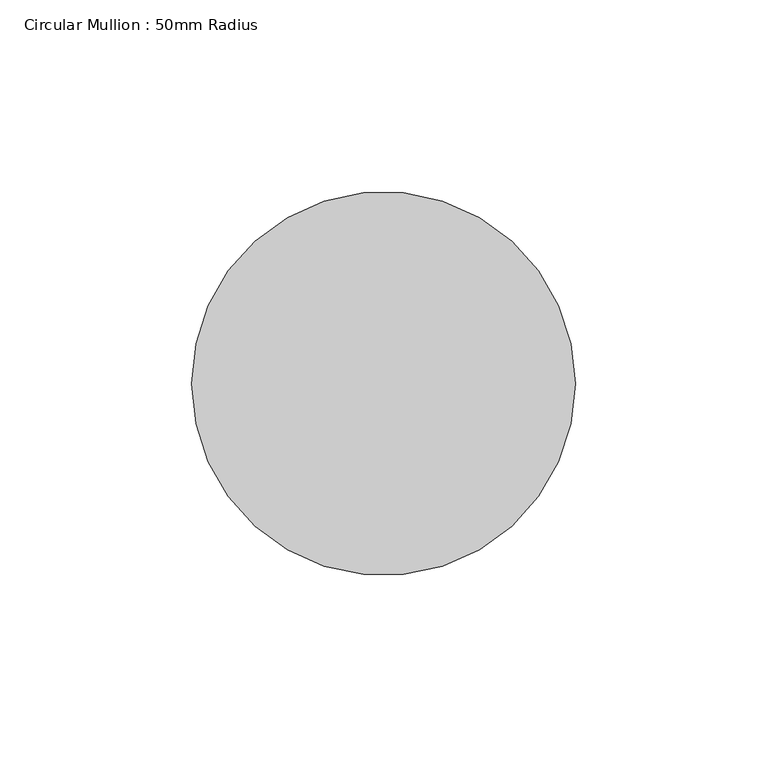
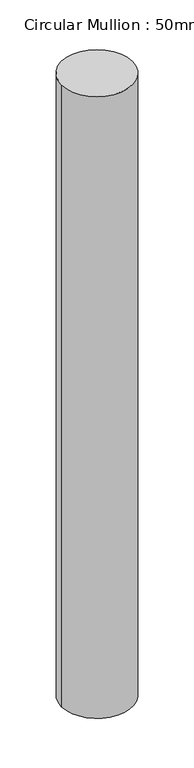
"""IFC4 building model written with IfcOpenShell, lengths in millimetres: member geometry, Circular Mullion : 50mm Radius."""

from ifc_helpers import new_model, si_unit, point, frame, origin, origin_2d, place, context, project, spatial, circle_curve, trimmed, segment, composite_curve, outline, extrude, source, transform, mapped, element, save


def circular_mullion_50mm_radius_75daf3a3(model_context):
    return source(origin(), model_context, "Body", "SweptSolid", [
        extrude(outline(composite_curve([segment(trimmed(circle_curve(origin_2d(), 50.0), [point((50.0, 0.0))], [point((-50.0, 0.0))], False, "CARTESIAN"), True, "CONTINUOUS"), segment(trimmed(circle_curve(origin_2d(), 50.0), [point((-50.0, 0.0))], [point((50.0, 0.0))], False, "CARTESIAN"), True, "CONTINUOUS")], self_intersect=False)), frame((0.0, 0.0, -926.1480661), z_axis=(0.0, 0.0, 1.0), x_axis=(1.0, 0.0, 0.0)), (0.0, 0.0, 1.0), 926.1480661),
    ])


if __name__ == "__main__":
    model = new_model("IFC4")
    model_context = context("Model", 3, world=origin())
    ifc_project = project(units=[si_unit("LENGTHUNIT", "METRE", prefix="MILLI")], contexts=[model_context])
    site = spatial("IfcSite", under=ifc_project)
    building = spatial("IfcBuilding", under=site)
    placement = place(None, origin())
    circular_mullion_50mm_radius_shape = circular_mullion_50mm_radius_75daf3a3(model_context)
    element("IfcMember", 1, ObjectType="Circular Mullion : 50mm Radius", at=placement, inside=building, context=model_context, shape_type="MappedRepresentation", body=[
        mapped(circular_mullion_50mm_radius_shape, transform((0.0, 0.0, 0.0), x_axis=(1.0, 0.0, 0.0), y_axis=(0.0, 1.0, 0.0), z_axis=(0.0, 0.0, 1.0))),
    ])
    save(model, "model.ifc")

# Revit data of these elements
# Type "Circular Mullion : 50mm Radius"
#   built-in parameter 1007350 = 0.164042 (stored number, unit not read)
# Element 1 (IfcMember, "Circular Mullion : 50mm Radius")
#   Materials on its faces: "Aluminium"
# Materials
#   "Aluminium": class "Metal", colour RGB 247 247 247, transparency 0, Description = "Aluminium 6061", Cost = 0
